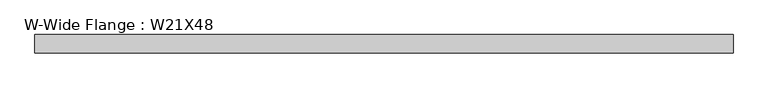
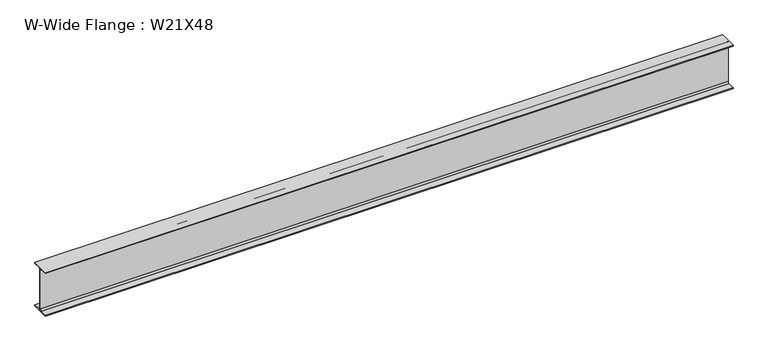
"""IFC4 building model written with IfcOpenShell, lengths in millimetres: beam geometry, W-Wide Flange : W21X48."""

from ifc_helpers import new_model, si_unit, point, frame, frame_2d, origin, place, context, project, spatial, polyline, circle_curve, trimmed, segment, composite_curve, outline, extrude, source, transform, mapped, element, save


def w_wide_flange_w21x48_70df18ae(model_context):
    return source(origin(), model_context, "Body", "SweptSolid", [
        extrude(outline(composite_curve([segment(polyline([(103.378, -250.698), (103.378, -261.62), (-103.378, -261.62), (-103.378, -250.698), (-22.098, -250.698)]), True, "CONTINUOUS"), segment(trimmed(circle_curve(frame_2d((-22.098, -233.045)), 17.653), [point((-22.098, -250.698))], [point((-4.445, -233.045))], True, "CARTESIAN"), True, "CONTINUOUS"), segment(polyline([(-4.445, -233.045), (-4.445, 233.045)]), True, "CONTINUOUS"), segment(trimmed(circle_curve(frame_2d((-22.098, 233.045)), 17.653), [point((-4.445, 233.045))], [point((-22.098, 250.698))], True, "CARTESIAN"), True, "CONTINUOUS"), segment(polyline([(-22.098, 250.698), (-103.378, 250.698), (-103.378, 261.62), (103.378, 261.62), (103.378, 250.698), (22.098, 250.698)]), True, "CONTINUOUS"), segment(trimmed(circle_curve(frame_2d((22.098, 233.045)), 17.653), [point((22.098, 250.698))], [point((4.445, 233.045))], True, "CARTESIAN"), True, "CONTINUOUS"), segment(polyline([(4.445, 233.045), (4.445, -233.045)]), True, "CONTINUOUS"), segment(trimmed(circle_curve(frame_2d((22.098, -233.045)), 17.653), [point((4.445, -233.045))], [point((22.098, -250.698))], True, "CARTESIAN"), True, "CONTINUOUS"), segment(polyline([(22.098, -250.698), (103.378, -250.698)]), True, "CONTINUOUS")], self_intersect=False)), frame((-3911.6, 0.0, 0.0), z_axis=(1.0, 0.0, 0.0), x_axis=(0.0, 1.0, 0.0)), (0.0, 0.0, 1.0), 7823.2),
    ])


if __name__ == "__main__":
    model = new_model("IFC4")
    model_context = context("Model", 3, world=origin())
    ifc_project = project(units=[si_unit("LENGTHUNIT", "METRE", prefix="MILLI")], contexts=[model_context])
    site = spatial("IfcSite", under=ifc_project)
    building = spatial("IfcBuilding", under=site)
    placement = place(None, origin())
    w_wide_flange_w21x48_shape = w_wide_flange_w21x48_70df18ae(model_context)
    element("IfcBeam", 1, ObjectType="W-Wide Flange : W21X48", at=placement, inside=building, context=model_context, shape_type="MappedRepresentation", body=[
        mapped(w_wide_flange_w21x48_shape, transform((0.0, 0.0, 0.0), x_axis=(1.0, 0.0, 0.0), y_axis=(0.0, 1.0, 0.0), z_axis=(0.0, 0.0, 1.0))),
    ])
    save(model, "model.ifc")

# Revit data of these elements
# Type "W-Wide Flange : W21X48"
#   Assembly Code = "B10"
#   W = 48
#   Length [instance default] = 5' - 0"
#   bf = 0' - 8.14"
#   d = 1' - 8.6"
#   k = 0' - 1 1/8"
#   k2 = 0' - 0.695"
#   tf = 0' - 0.43"
#   tw = 0' - 0.35"
#   A = 0.0979167 SF
#   Structural Material [instance default] = Steel ASTM A992
# Element 1 (IfcBeam, "W-Wide Flange : W21X48")
#   Materials on its faces: "Steel ASTM A992"
# Materials
#   "Steel ASTM A992": class "Metal", colour RGB 199 199 199, transparency 0, Description = "Structural steel 50ksi", Cost = 0
